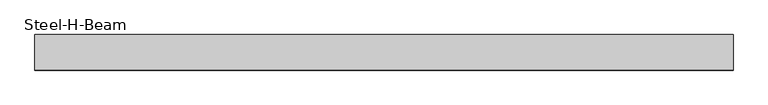
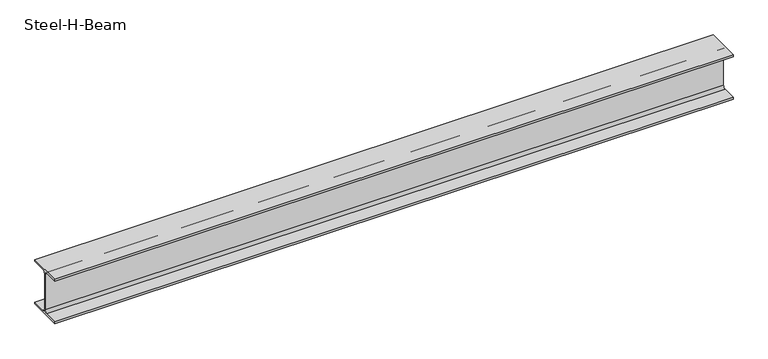
"""IFC4 building model written with IfcOpenShell, lengths in millimetres: beam geometry, Steel-H-Beam : BM121_H-340×250x9x14."""

import ifcopenshell
import ifcopenshell.guid

model = None  # the IFC model being written
_history = None  # IfcOwnerHistory: only IFC2X3 demands one
_inside = {}  # id of a spatial element -> (the spatial element, [elements in it])
_under = {}  # id of a project, library or spatial element -> (it, [spatial elements below it])
_declared = {}  # id of a project -> (the project, [libraries it declares])
_typed = {}  # id of a type object -> (the type object, [elements of that type])
_made_of = {}  # id of a material, layer set ... -> (it, [elements and type objects made of it])


def new_model(schema):
    """Start an empty IFC model of exactly this schema.

    Asked for "IFC4X3", IfcOpenShell would pick the latest addendum, in which some entities
    have other attributes; the version numbers below select the first issue.
    IFC2X3 requires an IfcOwnerHistory on every rooted entity: one is made here for all.
    """
    global model, _history
    if schema == "IFC4X3":
        model = ifcopenshell.file(schema_version=(4, 3, 0, 0))
    else:
        model = ifcopenshell.file(schema=schema)
    _inside.clear()
    _under.clear()
    _declared.clear()
    _typed.clear()
    _made_of.clear()
    _history = None
    if model.schema == "IFC2X3":
        org = make("IfcOrganization", Name="unknown")
        user = make(
            "IfcPersonAndOrganization",
            ThePerson=make("IfcPerson", FamilyName="unknown"),
            TheOrganization=org,
        )
        app = make(
            "IfcApplication",
            ApplicationDeveloper=org,
            Version="unknown",
            ApplicationFullName="unknown",
            ApplicationIdentifier="unknown",
        )
        _history = make(
            "IfcOwnerHistory",
            OwningUser=user,
            OwningApplication=app,
            ChangeAction="ADDED",
            CreationDate=0,
        )
    return model


def make(cls, **values):
    """One entity of the class cls with the attributes given. An attribute that is None is left unset."""
    return model.create_entity(
        cls, **{name: value for name, value in values.items() if value is not None}
    )


def rooted(cls, **values):
    """An entity with a GlobalId (a new one), such as an element, a storey or a relation."""
    return make(cls, GlobalId=ifcopenshell.guid.new(), OwnerHistory=_history, **values)


def si_unit(unit_type, name, prefix=None):
    """IfcSIUnit, for example si_unit("LENGTHUNIT", "METRE", prefix="MILLI")."""
    return make("IfcSIUnit", UnitType=unit_type, Prefix=prefix, Name=name)


def assignment(units):
    """IfcUnitAssignment: the units of a project."""
    return None if units is None else make("IfcUnitAssignment", Units=units)


def point(xyz):
    """IfcCartesianPoint."""
    return None if xyz is None else make("IfcCartesianPoint", Coordinates=xyz)


def direction(xyz):
    """IfcDirection."""
    return None if xyz is None else make("IfcDirection", DirectionRatios=xyz)


def frame(location, z_axis=None, x_axis=None):
    """IfcAxis2Placement3D, a coordinate frame: its origin and axes. An axis left out is left unset."""
    return make(
        "IfcAxis2Placement3D",
        Location=point(location),
        Axis=direction(z_axis),
        RefDirection=direction(x_axis),
    )


def frame_2d(location, x_axis=None):
    """IfcAxis2Placement2D, a coordinate frame in the plane: its origin and x axis."""
    return make(
        "IfcAxis2Placement2D", Location=point(location), RefDirection=direction(x_axis)
    )


def origin():
    """The frame at (0, 0, 0) with its axes left unset."""
    return frame((0.0, 0.0, 0.0))


def place(relative_to, where):
    """IfcLocalPlacement: puts the frame where relative to a parent placement (None: the world)."""
    return make(
        "IfcLocalPlacement", PlacementRelTo=relative_to, RelativePlacement=where
    )


def context(
    kind, dimensions, precision=None, world=None, true_north=None, identifier=None
):
    """IfcGeometricRepresentationContext, for example the 3D "Model" context."""
    return make(
        "IfcGeometricRepresentationContext",
        ContextIdentifier=identifier,
        ContextType=kind,
        CoordinateSpaceDimension=dimensions,
        Precision=precision,
        WorldCoordinateSystem=world,
        TrueNorth=true_north,
    )


def project(units=None, contexts=None):
    """IfcProject with its units and contexts."""
    return rooted(
        "IfcProject",
        Name="project",
        RepresentationContexts=contexts,
        UnitsInContext=assignment(units),
    )


def spatial(cls, under=None, at=None, **own):
    """A site, building, storey or space (cls), placed at a placement, below another one or the project."""
    s = rooted(cls, ObjectPlacement=at, **own)
    if under is not None:
        _under.setdefault(under.id(), (under, []))[1].append(s)
    return s


def polyline(points):
    """IfcPolyline through the points."""
    return make("IfcPolyline", Points=[point(p) for p in points])


def circle_curve(where, radius):
    """IfcCircle in the frame where."""
    return make("IfcCircle", Position=where, Radius=radius)


def trimmed(basis, trim1, trim2, sense, master):
    """IfcTrimmedCurve: the piece of a basis curve between two trims."""
    return make(
        "IfcTrimmedCurve",
        BasisCurve=basis,
        Trim1=trim1,
        Trim2=trim2,
        SenseAgreement=sense,
        MasterRepresentation=master,
    )


def segment(curve, same_sense, transition):
    """IfcCompositeCurveSegment."""
    return make(
        "IfcCompositeCurveSegment",
        Transition=transition,
        SameSense=same_sense,
        ParentCurve=curve,
    )


def composite_curve(segments, self_intersect=None):
    """IfcCompositeCurve: segments joined end to end."""
    return make("IfcCompositeCurve", Segments=segments, SelfIntersect=self_intersect)


def outline(outer, holes=None, kind="AREA"):
    """IfcArbitraryClosedProfileDef: a profile drawn as a closed curve; with holes, ...WithVoids."""
    if holes is None:
        return make("IfcArbitraryClosedProfileDef", ProfileType=kind, OuterCurve=outer)
    return make(
        "IfcArbitraryProfileDefWithVoids",
        ProfileType=kind,
        OuterCurve=outer,
        InnerCurves=holes,
    )


def extrude(swept, where, along, depth):
    """IfcExtrudedAreaSolid: the profile swept, set in the frame where, extruded along a direction by depth."""
    return make(
        "IfcExtrudedAreaSolid",
        SweptArea=swept,
        Position=where,
        ExtrudedDirection=direction(along),
        Depth=depth,
    )


def shape(context_of_items, identifier, shape_type, items):
    """IfcShapeRepresentation: the items that make up one representation, for example the "Body"."""
    return make(
        "IfcShapeRepresentation",
        ContextOfItems=context_of_items,
        RepresentationIdentifier=identifier,
        RepresentationType=shape_type,
        Items=items,
    )


def source(mapping_origin, context_of_items, identifier, shape_type, items):
    """IfcRepresentationMap: a shape defined once, which mapped items show again and again."""
    return make(
        "IfcRepresentationMap",
        MappingOrigin=mapping_origin,
        MappedRepresentation=shape(context_of_items, identifier, shape_type, items),
    )


def transform(
    local_origin,
    x_axis=None,
    y_axis=None,
    z_axis=None,
    scale=None,
    scale2=None,
    scale3=None,
    uniform=True,
):
    """IfcCartesianTransformationOperator3D, or its non-uniform kind. x_axis, y_axis, z_axis: its Axis1, 2, 3."""
    if uniform:
        return make(
            "IfcCartesianTransformationOperator3D",
            Axis1=direction(x_axis),
            Axis2=direction(y_axis),
            LocalOrigin=point(local_origin),
            Scale=scale,
            Axis3=direction(z_axis),
        )
    return make(
        "IfcCartesianTransformationOperator3DnonUniform",
        Axis1=direction(x_axis),
        Axis2=direction(y_axis),
        LocalOrigin=point(local_origin),
        Scale=scale,
        Axis3=direction(z_axis),
        Scale2=scale2,
        Scale3=scale3,
    )


def mapped(mapping_source, mapping_target):
    """IfcMappedItem: shows the shape of a source again, moved by a transform."""
    return make(
        "IfcMappedItem", MappingSource=mapping_source, MappingTarget=mapping_target
    )


def made_of(thing, what):
    """Note that an element or type object is made of a material, layer set ...; save() writes the relation."""
    if what is not None:
        _made_of.setdefault(what.id(), (what, []))[1].append(thing)
    return thing


def element(
    cls,
    number,
    at=None,
    inside=None,
    cuts=None,
    type_object=None,
    material=None,
    context=None,
    identifier="Body",
    shape_type=None,
    held_by="IfcProductDefinitionShape",
    body=None,
    shapes=None,
    **own,
):
    """One element of the class cls, such as IfcWall. Its Tag is "e" and its number.

    at: its placement. inside: the storey or other place that contains it. cuts: it is an
    opening in that element (IfcRelVoidsElement). A single representation is given by context,
    identifier, shape_type and body (its items); several are given by shapes. held_by: the class
    of the entity that holds the representations. save() writes the other relations.
    """
    e = rooted(cls, Tag="e%d" % number, ObjectPlacement=at, **own)
    if body is not None:
        shapes = [shape(context, identifier, shape_type, body)]
    if shapes is not None:
        e.Representation = make(held_by, Representations=shapes)
    if inside is not None:
        _inside.setdefault(inside.id(), (inside, []))[1].append(e)
    if cuts is not None:
        rooted(
            "IfcRelVoidsElement", RelatingBuildingElement=cuts, RelatedOpeningElement=e
        )
    if type_object is not None:
        _typed.setdefault(type_object.id(), (type_object, []))[1].append(e)
    return made_of(e, material)


def aggregate(whole, parts):
    """IfcRelAggregates: a whole, such as a stair, and the parts it consists of."""
    return rooted("IfcRelAggregates", RelatingObject=whole, RelatedObjects=parts)


def save(model, path):
    """Write the relations noted so far, then the file.

    IfcRelAggregates (storeys below a building ...), IfcRelContainedInSpatialStructure (elements
    in a storey), IfcRelDefinesByType, IfcRelAssociatesMaterial and IfcRelDeclares: one each for
    every whole, place, type object, material and project.
    """
    for whole, parts in _under.values():
        aggregate(whole, parts)
    for where, things in _inside.values():
        rooted(
            "IfcRelContainedInSpatialStructure",
            RelatedElements=things,
            RelatingStructure=where,
        )
    for kind, things in _typed.values():
        rooted("IfcRelDefinesByType", RelatedObjects=things, RelatingType=kind)
    for what, things in _made_of.values():
        rooted("IfcRelAssociatesMaterial", RelatedObjects=things, RelatingMaterial=what)
    for by, libraries in _declared.values():
        rooted("IfcRelDeclares", RelatingContext=by, RelatedDefinitions=libraries)
    model.write(path)


def steel_h_beam_5215ea41(model_context):
    return source(origin(), model_context, "Body", "SweptSolid", [
        extrude(outline(composite_curve([segment(polyline([(-125.0, -156.0), (-24.5, -156.0)]), True, "CONTINUOUS"), segment(trimmed(circle_curve(frame_2d((-24.5, -136.0)), 20.0), [point((-24.5, -156.0))], [point((-4.5, -136.0))], True, "CARTESIAN"), True, "CONTINUOUS"), segment(polyline([(-4.5, -136.0), (-4.5, 136.0)]), True, "CONTINUOUS"), segment(trimmed(circle_curve(frame_2d((-24.5, 136.0)), 20.0), [point((-4.5, 136.0))], [point((-24.5, 156.0))], True, "CARTESIAN"), True, "CONTINUOUS"), segment(polyline([(-24.5, 156.0), (-125.0, 156.0), (-125.0, 170.0), (125.0, 170.0), (125.0, 156.0), (24.5, 156.0)]), True, "CONTINUOUS"), segment(trimmed(circle_curve(frame_2d((24.5, 136.0)), 20.0), [point((24.5, 156.0))], [point((4.5, 136.0))], True, "CARTESIAN"), True, "CONTINUOUS"), segment(polyline([(4.5, 136.0), (4.5, -136.0)]), True, "CONTINUOUS"), segment(trimmed(circle_curve(frame_2d((24.5, -136.0)), 20.0), [point((4.5, -136.0))], [point((24.5, -156.0))], True, "CARTESIAN"), True, "CONTINUOUS"), segment(polyline([(24.5, -156.0), (125.0, -156.0), (125.0, -170.0), (-125.0, -170.0), (-125.0, -156.0)]), True, "CONTINUOUS")], self_intersect=False)), frame((-2363.9803034, 0.0, 0.0), z_axis=(1.0, 0.0, 0.0), x_axis=(0.0, 1.0, 0.0)), (0.0, 0.0, 1.0), 4905.0160952),
    ])


if __name__ == "__main__":
    model = new_model("IFC4")
    model_context = context("Model", 3, world=origin())
    ifc_project = project(units=[si_unit("LENGTHUNIT", "METRE", prefix="MILLI")], contexts=[model_context])
    site = spatial("IfcSite", under=ifc_project)
    building = spatial("IfcBuilding", under=site)
    placement = place(None, origin())
    steel_h_beam_shape = steel_h_beam_5215ea41(model_context)
    element("IfcBeam", 1, ObjectType="Steel-H-Beam : BM121_H-340×250x9x14", at=placement, inside=building, context=model_context, shape_type="MappedRepresentation", body=[
        mapped(steel_h_beam_shape, transform((0.0, 0.0, 0.0), x_axis=(1.0, 0.0, 0.0), y_axis=(0.0, 1.0, 0.0), z_axis=(0.0, 0.0, 1.0))),
    ])
    save(model, "model.ifc")

# Revit data of these elements
# Type "Steel-H-Beam : BM121_H-340×250x9x14"
#   Surface Area = 0.00 m²/m
#   Section Area = 101.5 cm²
#   Mass per Unit Length = 79.70 kg/m
#   Length [instance default] = 1524 mm
#   B = 250 mm
#   H = 340 mm
#   r = 20 mm
#   tw = 9 mm
#   tf = 14 mm
#   hec_material4 [instance default] = none
#   hec_material3 [instance default] = none
#   hec_material2 [instance default] = none
#   hec_material1 [instance default] = none
#   Structural Material [instance default] = Steel, 45-345
#   Assembly Code = ""
# Element 1 (IfcBeam, "Steel-H-Beam : BM121_H-340×250x9x14")
#   hec_material4 = S01AA010-00002_Main Steel Structure Fabrication Work_Shelter/Building_Steel Painting/Coating_for Fireproofed Steel Surface, Surface Preparation & Primer Coat
#   hec_material3 = F01AC000-00002_Building/Shelter Fire Proofing Work_Intumescent Coating Type_1 hr. rating (UL 1709))
#   hec_material2 = S01AA010-00001_Main Steel Structure Fabrication Work_Shelter/Building_Steel Painting/Coating_for Non-Fireproofed Steel Surface, Surface Preparation, Primer, Second & Final Coat
#   hec_material1 = S03AA028-00001_Main Steel Structure Erection Work_Shelter/Building_Medium Steel
#   Materials on its faces: "Steel, 45-345"
# Materials
#   "Steel, 45-345": class "Metal", colour RGB 189 187 185, transparency 0, Description = "Steel 345 MPa", Cost = 0
#   "S01AA010-00002_Main Steel Structure Fabrication Work_Shelter/Building_Steel Painting/Coating_for Fireproofed Steel Surface, Surface Preparation & Primer Coat": class "Metal", colour RGB 120 120 120, transparency 0, Description = "Paint finished steel", W00) Work Master Code = "SS01AA010-00002", W01) Work Master_Lv1 = "Main Steel Structure Fabrication Work", W02) Work Master_Lv2 = "Shelter/Building", W03) Work Master_Spec.1 = "Steel Painting/Coating", W04) Work Master_Spec.2 = "for Fireproofed Steel Surface, Surface Preparation & Primer Coat", Cost = 0
#   "F01AC000-00002_Building/Shelter Fire Proofing Work_Intumescent Coating Type_1 hr. rating (UL 1709))": class "Metal", colour RGB 255 128 128, transparency 0, Description = "Paint finished steel", W00) Work Master Code = "F01AC000-00002", W01) Work Master_Lv1 = "Building/Shelter Fire Proofing Work", W02) Work Master_Lv2 = "Intumescent Coating Type", W03) Work Master_Spec.1 = "1 hr. rating (UL 1709)", Cost = 0
#   "S01AA010-00001_Main Steel Structure Fabrication Work_Shelter/Building_Steel Painting/Coating_for Non-Fireproofed Steel Surface, Surface Preparation, Primer, Second & Final Coat": class "Metal", colour RGB 120 120 120, transparency 0, Description = "Paint finished steel", W00) Work Master Code = "S01AA010-00001", W01) Work Master_Lv1 = "Main Steel Structure Fabrication Work", W02) Work Master_Lv2 = "Shelter/Building", W03) Work Master_Spec.1 = "Steel Painting/Coating", W04) Work Master_Spec.2 = "for Non-Fireproofed Steel Surface, Surface Preparation, Primer, Second & Final Coat", Cost = 0
#   "S03AA028-00001_Main Steel Structure Erection Work_Shelter/Building_Medium Steel": class "Metal", colour RGB 120 120 120, transparency 0, Comments = "(90KG/M>Weight≥30KG/M)", Description = "Structural steel 50ksi", W00) Work Master Code = "S03AA028-0001", W01) Work Master_Lv1 = "Main Steel Structure Erection Work", W02) Work Master_Lv2 = "Shelter/Building", W03) Work Master_Spec.1 = "Medium Steel (90KG/M>Weight≥30KG/M)", Cost = 0
